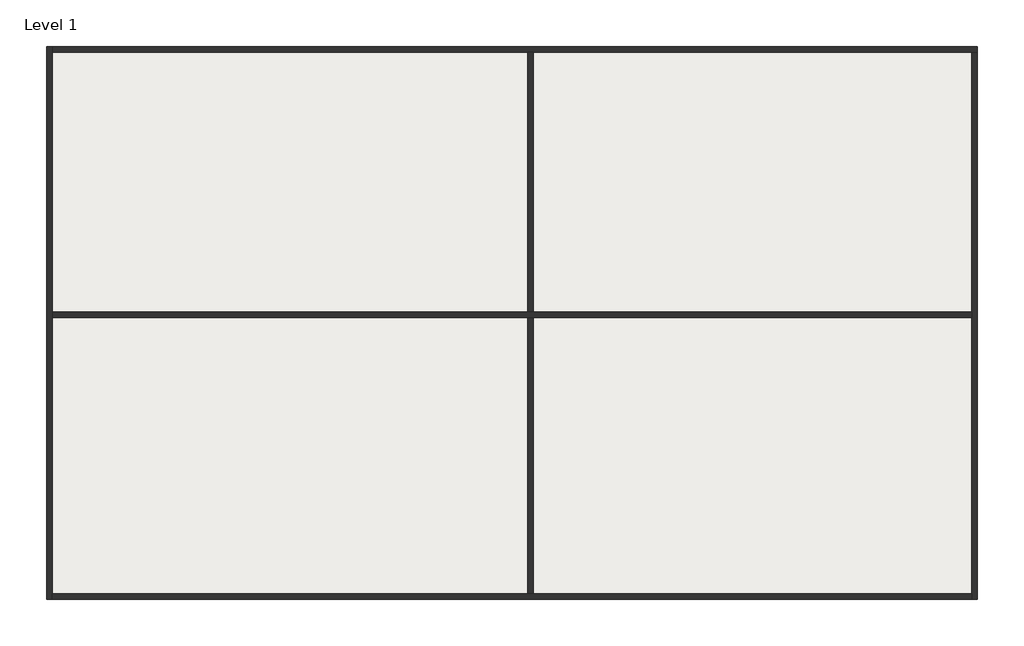
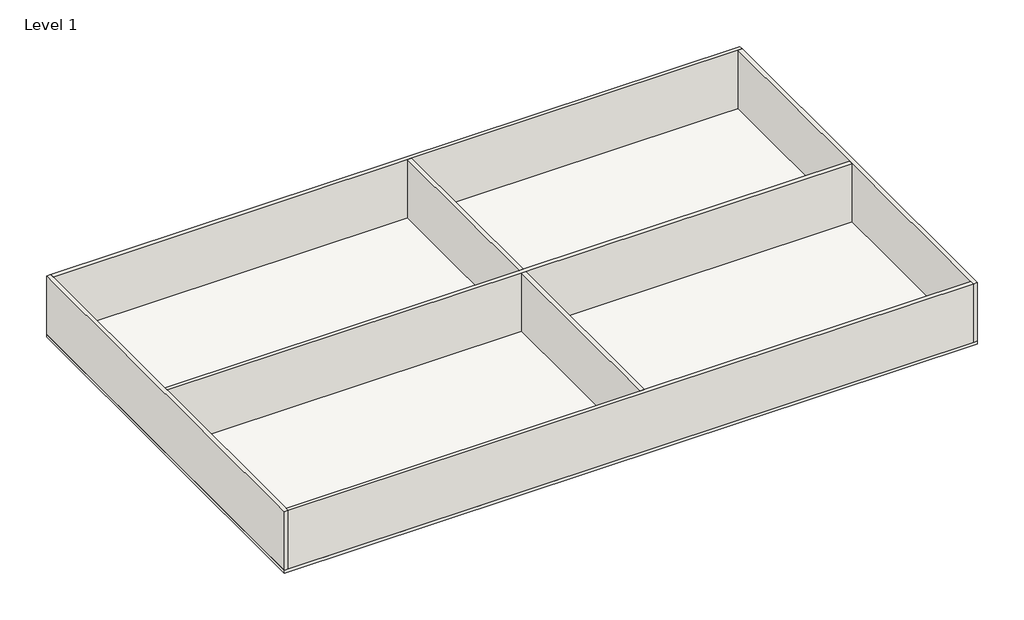
# One storey: 6 walls, 1 slab.
"""IFC4 building model written with IfcOpenShell, lengths in millimetres."""

from ifc_helpers import new_model, si_unit, frame, origin, origin_with_axes, place, context, project, spatial, polyline, outline, extrude, faceted_brep, element, save

model = new_model("IFC4")

# Units and contexts
model_context = context("Model", 3, world=origin())
ifc_project = project(units=[si_unit("LENGTHUNIT", "METRE", prefix="MILLI")], contexts=[model_context])

# Site, building, storey
site = spatial("IfcSite", under=ifc_project)
building = spatial("IfcBuilding", under=site)
storey = spatial("IfcBuildingStorey", under=building, Name="Level 1", Elevation=0.0)

# Slab
placement = place(None, origin())
element("IfcSlab", 1, ObjectType="Concrete Slab - 6\"", at=placement, inside=storey, context=model_context, shape_type="SweptSolid", body=[
    extrude(outline(polyline([(-3502.1882593, 10794.88673), (30686.2117407, 10794.88673), (30686.2117407, -9525.11327), (-3502.1882593, -9525.11327), (-3502.1882593, 10794.88673)])), frame((0.0, 0.0, -152.4), z_axis=(0.0, 0.0, 1.0), x_axis=(1.0, 0.0, 0.0)), (0.0, 0.0, 1.0), 152.4),
])

# Walls
element("IfcWall", 2, ObjectType="Generic - 8\"", at=placement, inside=storey, context=model_context, shape_type="Brep", body=[
    faceted_brep([(-3298.9882593, -9525.11327, 0.0), (-3298.9882593, -9321.91327, 0.0), (-3298.9882593, 838.08673, 0.0), (-3298.9882593, 1041.28673, 0.0), (-3298.9882593, 10591.68673, 0.0), (-3298.9882593, 10794.88673, 0.0), (-3298.9882593, 10794.88673, 3048.0), (-3298.9882593, 10591.68673, 3048.0), (-3298.9882593, 1041.28673, 3048.0), (-3298.9882593, 838.08673, 3048.0), (-3298.9882593, -9321.91327, 3048.0), (-3298.9882593, -9525.11327, 3048.0), (-3502.1882593, -9525.11327, 0.0), (-3502.1882593, -9525.11327, 3048.0), (-3502.1882593, 10794.88673, 3048.0), (-3502.1882593, 10794.88673, 0.0)], [[[0, 1, 2, 3, 4, 5, 6, 7, 8, 9, 10, 11]], [[12, 13, 14, 15]], [[5, 4, 3, 2, 1, 0, 12, 15]], [[11, 10, 9, 8, 7, 6, 14, 13]], [[6, 5, 15, 14]], [[0, 11, 13, 12]]]),
])
element("IfcWall", 3, ObjectType="Generic - 8\"", at=placement, inside=storey, context=model_context, shape_type="Brep", body=[
    faceted_brep([(-3298.9882593, 10591.68673, 0.0), (14176.2117407, 10591.68673, 0.0), (14379.4117407, 10591.68673, 0.0), (30483.0117407, 10591.68673, 0.0), (30686.2117407, 10591.68673, 0.0), (30686.2117407, 10591.68673, 3048.0), (30483.0117407, 10591.68673, 3048.0), (14379.4117407, 10591.68673, 3048.0), (14176.2117407, 10591.68673, 3048.0), (-3298.9882593, 10591.68673, 3048.0), (-3298.9882593, 10794.88673, 0.0), (-3298.9882593, 10794.88673, 3048.0), (30686.2117407, 10794.88673, 3048.0), (30686.2117407, 10794.88673, 0.0)], [[[0, 1, 2, 3, 4, 5, 6, 7, 8, 9]], [[10, 11, 12, 13]], [[4, 3, 2, 1, 0, 10, 13]], [[9, 8, 7, 6, 5, 12, 11]], [[0, 9, 11, 10]], [[5, 4, 13, 12]]]),
])
element("IfcWall", 4, ObjectType="Generic - 8\"", at=placement, inside=storey, context=model_context, shape_type="Brep", body=[
    faceted_brep([(30483.0117407, 10591.68673, 0.0), (30483.0117407, 1041.28673, 0.0), (30483.0117407, 838.08673, 0.0), (30483.0117407, -9321.91327, 0.0), (30483.0117407, -9525.11327, 0.0), (30483.0117407, -9525.11327, 3048.0), (30483.0117407, -9321.91327, 3048.0), (30483.0117407, 838.08673, 3048.0), (30483.0117407, 1041.28673, 3048.0), (30483.0117407, 10591.68673, 3048.0), (30686.2117407, 10591.68673, 0.0), (30686.2117407, 10591.68673, 3048.0), (30686.2117407, -9525.11327, 3048.0), (30686.2117407, -9525.11327, 0.0)], [[[0, 1, 2, 3, 4, 5, 6, 7, 8, 9]], [[10, 11, 12, 13]], [[4, 3, 2, 1, 0, 10, 13]], [[9, 8, 7, 6, 5, 12, 11]], [[0, 9, 11, 10]], [[5, 4, 13, 12]]]),
])
element("IfcWall", 5, ObjectType="Generic - 8\"", at=placement, inside=storey, context=model_context, shape_type="Brep", body=[
    faceted_brep([(30483.0117407, -9321.91327, 0.0), (14379.4117407, -9321.91327, 0.0), (14176.2117407, -9321.91327, 0.0), (-3298.9882593, -9321.91327, 0.0), (-3298.9882593, -9321.91327, 3048.0), (14176.2117407, -9321.91327, 3048.0), (14379.4117407, -9321.91327, 3048.0), (30483.0117407, -9321.91327, 3048.0), (30483.0117407, -9525.11327, 0.0), (30483.0117407, -9525.11327, 3048.0), (-3298.9882593, -9525.11327, 3048.0), (-3298.9882593, -9525.11327, 0.0)], [[[0, 1, 2, 3, 4, 5, 6, 7]], [[8, 9, 10, 11]], [[3, 2, 1, 0, 8, 11]], [[7, 6, 5, 4, 10, 9]], [[0, 7, 9, 8]], [[4, 3, 11, 10]]]),
])
element("IfcWall", 6, ObjectType="Generic - 8\"", at=placement, inside=storey, context=model_context, shape_type="Brep", body=[
    faceted_brep([(-3298.9882593, 838.08673, 0.0), (14176.2117407, 838.08673, 0.0), (14379.4117407, 838.08673, 0.0), (30483.0117407, 838.08673, 0.0), (30483.0117407, 838.08673, 3048.0), (14379.4117407, 838.08673, 3048.0), (14176.2117407, 838.08673, 3048.0), (-3298.9882593, 838.08673, 3048.0), (-3298.9882593, 1041.28673, 0.0), (-3298.9882593, 1041.28673, 3048.0), (14176.2117407, 1041.28673, 3048.0), (14379.4117407, 1041.28673, 3048.0), (30483.0117407, 1041.28673, 3048.0), (30483.0117407, 1041.28673, 0.0), (14379.4117407, 1041.28673, 0.0), (14176.2117407, 1041.28673, 0.0)], [[[0, 1, 2, 3, 4, 5, 6, 7]], [[8, 9, 10, 11, 12, 13, 14, 15]], [[3, 2, 1, 0, 8, 15, 14, 13]], [[7, 6, 5, 4, 12, 11, 10, 9]], [[0, 7, 9, 8]], [[4, 3, 13, 12]]]),
])
element("IfcWall", 7, ObjectType="Generic - 8\"", at=placement, inside=storey, context=model_context, shape_type="SweptSolid", body=[
    extrude(outline(polyline([(14176.2117407, 10591.68673), (14379.4117407, 10591.68673), (14379.4117407, 1041.28673), (14176.2117407, 1041.28673), (14176.2117407, 10591.68673)])), origin_with_axes(), (0.0, 0.0, 1.0), 3048.0),
    extrude(outline(polyline([(14379.4117407, -9321.91327), (14176.2117407, -9321.91327), (14176.2117407, 838.08673), (14379.4117407, 838.08673), (14379.4117407, -9321.91327)])), origin_with_axes(), (0.0, 0.0, 1.0), 3048.0),
])

save(model, "model.ifc")

# Revit data of these elements
# Project information
#   Project Issue Date = "Issue Date"
#   Project Status = "Project Status"
#   Client Name = "Owner"
#   Project Address = "Enter address here"
#   Project Name = "Project Name"
#   Project Number = "Project Number"
# Type "Concrete Slab - 6\""
#   Assembly Code = "B1010"
#   Function = 0
#   Layers, outside or top first: 0' - 6" "Concrete, Cast-in-Place gray" (function 1)
# Type "Generic - 8\""
#   Assembly Code = "B2010"
#   Layers, outside or top first: 0' - 8" no material (function 1)
# Element 1 (IfcSlab, "Concrete Slab - 6\"")
#   built-in parameter 1001955 = 1.5708 (stored number, unit not read)
#   Height Offset From Level = 0' - 0"
#   Phase Created = Project Completion
#   Materials on its faces: "Concrete, Cast-in-Place gray"
# Elements 2, 3, 4, 5, 6, 7 (IfcWall, "Generic - 8\"")
#   Top Offset = 0' - 0"
#   Base Offset = 0' - 0"
#   wall height = 10' - 0"
#   Phase Created = Project Completion
#   Base Constraint = Level 1
#   Top Constraint = Level 2
#   Materials on its faces: "Default Wall"
# Materials
#   "Concrete, Cast-in-Place gray": class "Concrete", colour RGB 192 192 192, transparency 0, Description = "Cast-in-place concrete", Cost = 0
#   "Default Wall": class "Miscellaneous", colour RGB 128 128 128, transparency 0, Cost = 0
# Space at (3588.172, 4695.298) mm, phase "Project Completion", upper level "Level 2", upper offset 0' - 0", lower offset 0' - 0"
#   Number = "1"
#   Name = "Space"
#   Actual Lighting Load per area = 0
#   Actual Power Load per area = 0
#   Sensible Heat Gain per person = 378.551 (stored number, unit not read)
#   Specified Lighting Load = 38654.2 (stored number, unit not read)
#   Specified Power Load = 38673.5 (stored number, unit not read)
#   Specified Lighting Load per area = 21.5171 (stored number, unit not read)
#   Specified Power Load per area = 21.5278 (stored number, unit not read)
#   Latent Heat Gain per person = 378.551 (stored number, unit not read)
#   Total Heat Gain per person = 0
#   Area per Person = 25 (stored number, unit not read)
#   Number of People = 71.8578 (stored number, unit not read)
#   Lighting Load Units = 0
#   Power Load Units = 0
#   Return Airflow = 0
#   Occupancy Unit = 1
#   Condition Type = 2
#   Construction Type = none
# Space at (21967.176, 4695.298) mm, phase "Project Completion", upper level "Level 2", upper offset 0' - 0", lower offset 0' - 0"
#   Number = "2"
#   Name = "Space"
#   Actual Lighting Load per area = 0
#   Actual Power Load per area = 0
#   Sensible Heat Gain per person = 0
#   Specified Lighting Load = 16037.2 (stored number, unit not read)
#   Specified Power Load = 9622.29 (stored number, unit not read)
#   Latent Heat Gain per person = 0
#   Total Heat Gain per person = 0
#   Area per Person = 0
#   Number of People = 107.657 (stored number, unit not read)
#   Lighting Load Units = 0
#   Power Load Units = 0
#   Return Airflow = 0
#   Occupancy Unit = -1
#   Condition Type = 2
#   Construction Type = none
# Space at (22075.928, -4602.956) mm, phase "Project Completion", upper level "Level 2", upper offset 0' - 0", lower offset 0' - 0"
#   Number = "3"
#   Name = "Space"
#   Actual Lighting Load per area = 0
#   Actual Power Load per area = 0
#   Sensible Heat Gain per person = 0
#   Specified Lighting Load = 18956.4 (stored number, unit not read)
#   Specified Power Load = 24643.4 (stored number, unit not read)
#   Latent Heat Gain per person = 0
#   Total Heat Gain per person = 0
#   Area per Person = 0
#   Number of People = 5.72644 (stored number, unit not read)
#   Lighting Load Units = 0
#   Power Load Units = 0
#   Return Airflow = 0
#   Occupancy Unit = -1
#   Condition Type = 2
#   Construction Type = none
